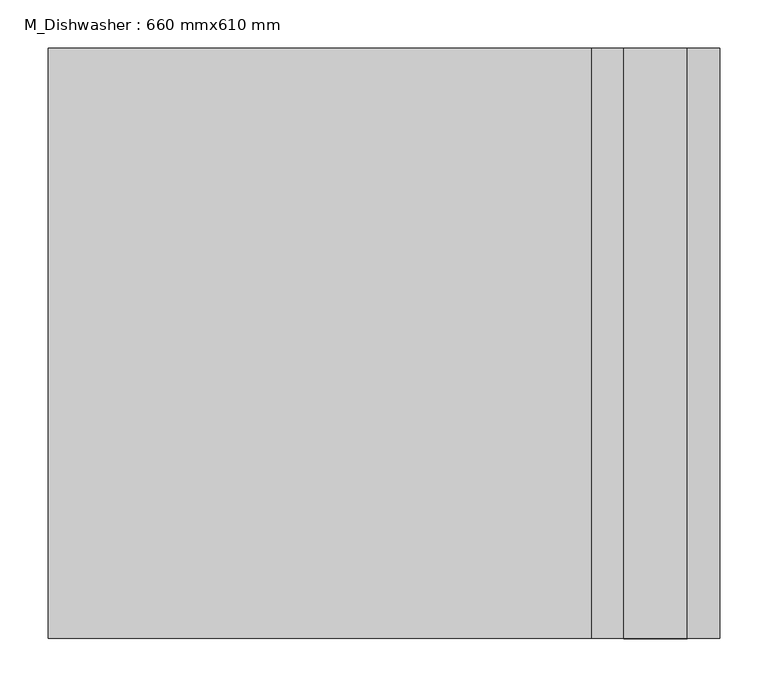
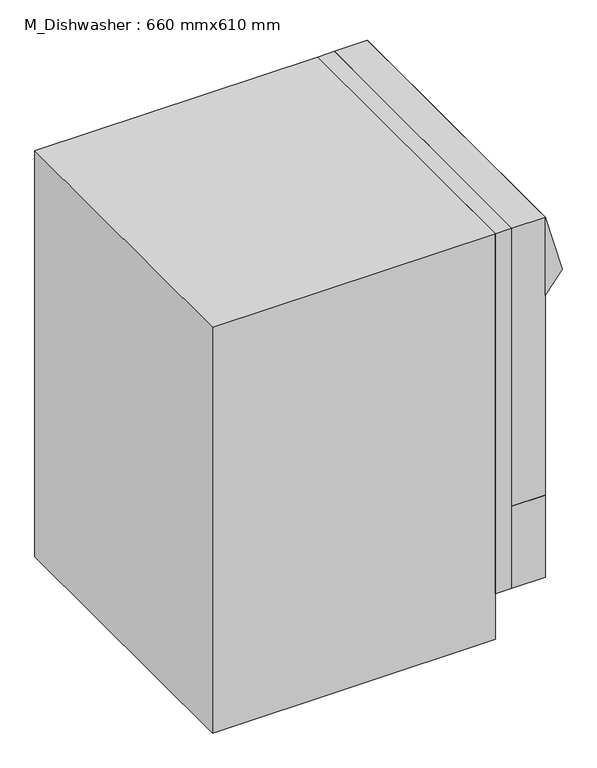
"""IFC4 building model written with IfcOpenShell, lengths in millimetres: flow terminal geometry, M_Dishwasher : 660 mmx610 mm."""

from ifc_helpers import new_model, si_unit, frame, origin, origin_with_axes, place, context, project, spatial, polyline, outline, extrude, source, transform, mapped, element, save


def m_dishwasher_660_mmx610_mm_c472654d(model_context):
    return source(origin(), model_context, "Body", "SweptSolid", [
        extrude(outline(polyline([(660.0, -305.0), (594.11875, -305.0), (594.11875, 305.0), (660.0, 305.0), (660.0, -305.0)])), frame((0.0, 0.0, 95.25), z_axis=(0.0, 0.0, 1.0), x_axis=(1.0, 0.0, 0.0)), (0.0, 0.0, 1.0), 172.24375),
        extrude(outline(polyline([(560.78125, 305.0), (560.78125, -305.0), (0.0, -305.0), (0.0, 305.0), (560.78125, 305.0)])), origin_with_axes(), (0.0, 0.0, 1.0), 850.0),
        extrude(outline(polyline([(729.35, 693.3375), (850.0, 660.0), (685.69375, 660.0), (729.35, 693.3375)])), frame((0.0, -305.0, 0.0), z_axis=(0.0, 1.0, 0.0), x_axis=(0.0, 0.0, 1.0)), (0.0, 0.0, 1.0), 610.0),
        extrude(outline(polyline([(660.0, -305.0), (594.11875, -305.0), (594.11875, 305.0), (660.0, 305.0), (660.0, -305.0)])), frame((0.0, 0.0, 267.49375), z_axis=(0.0, 0.0, 1.0), x_axis=(1.0, 0.0, 0.0)), (0.0, 0.0, 1.0), 582.50625),
        extrude(outline(polyline([(594.11875, -305.0), (560.78125, -305.0), (560.78125, 305.0), (594.11875, 305.0), (594.11875, -305.0)])), frame((0.0, 0.0, 95.25), z_axis=(0.0, 0.0, 1.0), x_axis=(1.0, 0.0, 0.0)), (0.0, 0.0, 1.0), 754.75),
    ])


if __name__ == "__main__":
    model = new_model("IFC4")
    model_context = context("Model", 3, world=origin())
    ifc_project = project(units=[si_unit("LENGTHUNIT", "METRE", prefix="MILLI")], contexts=[model_context])
    site = spatial("IfcSite", under=ifc_project)
    building = spatial("IfcBuilding", under=site)
    placement = place(None, origin())
    m_dishwasher_660_mmx610_mm_shape = m_dishwasher_660_mmx610_mm_c472654d(model_context)
    element("IfcFlowTerminal", 1, ObjectType="M_Dishwasher : 660 mmx610 mm", at=placement, inside=building, context=model_context, shape_type="MappedRepresentation", body=[
        mapped(m_dishwasher_660_mmx610_mm_shape, transform((0.0, 0.0, 0.0), x_axis=(1.0, 0.0, 0.0), y_axis=(0.0, 1.0, 0.0), z_axis=(0.0, 0.0, 1.0))),
    ])
    save(model, "model.ifc")

# Revit data of these elements
# Type "M_Dishwasher : 660 mmx610 mm"
#   HP = "0.5"
#   Sanitary Radius = 25 mm
#   Sanitary Diameter = 50 mm
#   WFU = 2
#   Voltage = 120 V
#   Overall Width = 2' - 0.01575"
#   Overall Length = 2' - 1.98425"
#   Overall Height = 2' - 9.46457"
#   Hot Water Radius = 7.5 mm
#   Hot Water Diameter = 15 mm
#   HWFU = 1.4
#   Flow Pressure [instance default] = 55158.0 Pa
#   Cold Water Radius = 7.5 mm
#   Cold Water Diameter = 15 mm
#   Apparent Load = 1090 VA
#   Number of Poles = 1
#   Load Classification = Appliance - Dwelling Unit
#   Dishwasher Material = none
#   Default Elevation = 0
#   CWFU = 0
